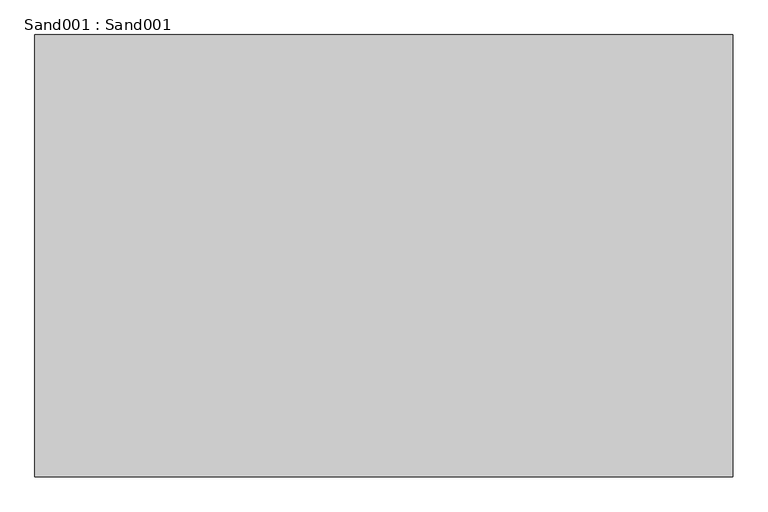
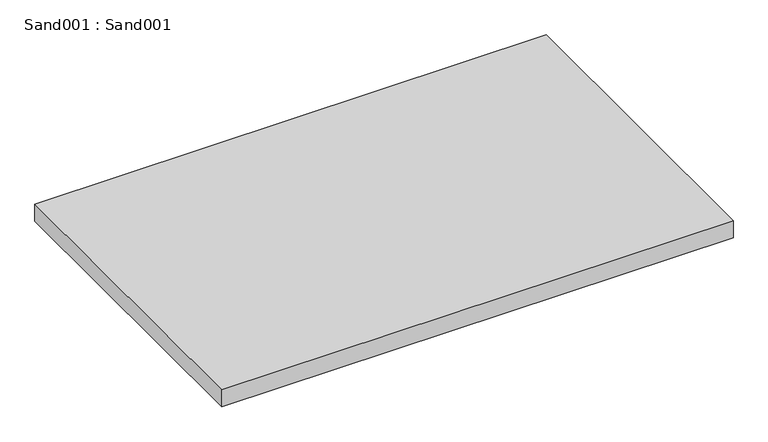
"""IFC4 building model written with IfcOpenShell, lengths in millimetres: proxy geometry, Sand001 : Sand001."""

from ifc_helpers import new_model, si_unit, frame, origin, place, context, project, spatial, polyline, outline, extrude, source, transform, mapped, element, save


def sand001_sand001_7a3855e9(model_context):
    return source(origin(), model_context, "Body", "SweptSolid", [
        extrude(outline(polyline([(14383.0178845, -4637.5417972), (14383.0178845, -5904.2981766), (12383.0178845, -5904.2981766), (12383.0178845, -4637.5417972), (14383.0178845, -4637.5417972)])), frame((0.0, 0.0, 36105.4523605), z_axis=(0.0, 0.0, 1.0), x_axis=(1.0, 0.0, 0.0)), (0.0, 0.0, 1.0), 70.2358801),
    ])


if __name__ == "__main__":
    model = new_model("IFC4")
    model_context = context("Model", 3, world=origin())
    ifc_project = project(units=[si_unit("LENGTHUNIT", "METRE", prefix="MILLI")], contexts=[model_context])
    site = spatial("IfcSite", under=ifc_project)
    building = spatial("IfcBuilding", under=site)
    placement = place(None, origin())
    sand001_sand001_shape = sand001_sand001_7a3855e9(model_context)
    element("IfcBuildingElementProxy", 1, Name="Sand001 : Sand001", ObjectType="Sand001 : Sand001", at=placement, inside=building, context=model_context, shape_type="MappedRepresentation", body=[
        mapped(sand001_sand001_shape, transform((0.0, 0.0, 0.0), x_axis=(1.0, 0.0, 0.0), y_axis=(0.0, 1.0, 0.0), z_axis=(0.0, 0.0, 1.0))),
    ])
    save(model, "model.ifc")

# Revit data of these elements
# Type "Sand001 : Sand001"
#   NameOverride = "Sand001"
# Element 1 (IfcBuildingElementProxy, "Sand001 : Sand001")
#   Materials on its faces: "2\" SAND LAYER"
# Materials
#   "2\" SAND LAYER": class "Unassigned", colour RGB 239 206 153, transparency 0, Cost = 0
